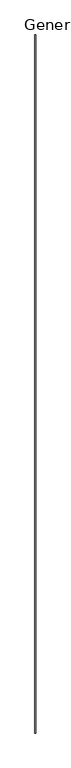
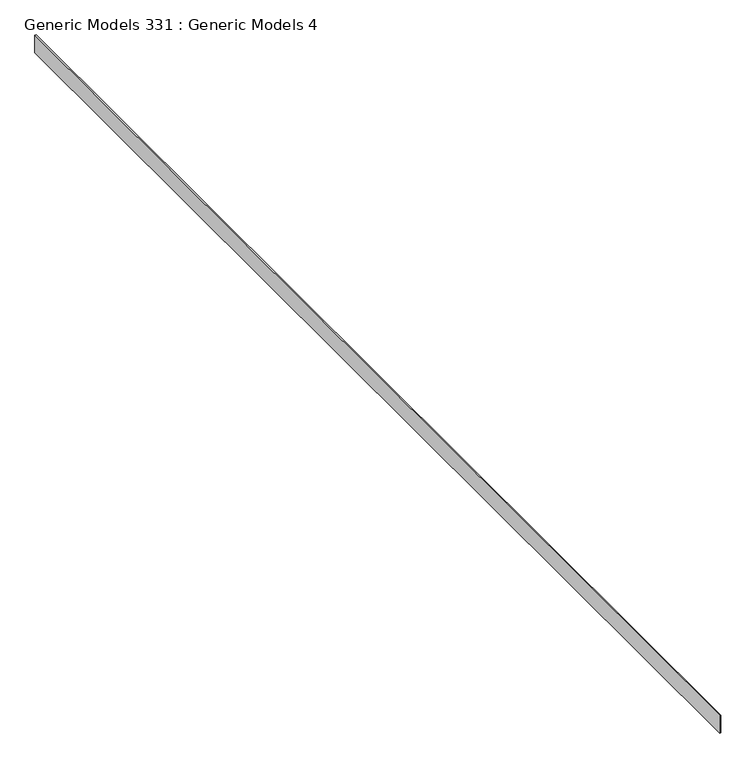
"""IFC4 building model written with IfcOpenShell, lengths in millimetres: proxy geometry, Generic Models 331 : Generic Models 4."""

from ifc_helpers import new_model, si_unit, frame, origin, place, context, project, spatial, polyline, outline, extrude, source, transform, mapped, element, save


def generic_models_331_generic_models_4_b2be233a(model_context):
    return source(origin(), model_context, "Body", "SweptSolid", [
        extrude(outline(polyline([(26420.1627812, 26848.7591064), (26401.1127812, 26848.7591064), (26401.1127812, 45492.3591064), (26420.1627812, 45492.3591064), (26420.1627812, 26848.7591064)])), frame((0.0, 0.0, 130596.677731), z_axis=(0.0, 0.0, 1.0), x_axis=(1.0, 0.0, 0.0)), (0.0, 0.0, 1.0), 293.6073068),
    ])


if __name__ == "__main__":
    model = new_model("IFC4")
    model_context = context("Model", 3, world=origin())
    ifc_project = project(units=[si_unit("LENGTHUNIT", "METRE", prefix="MILLI")], contexts=[model_context])
    site = spatial("IfcSite", under=ifc_project)
    building = spatial("IfcBuilding", under=site)
    placement = place(None, origin())
    generic_models_331_generic_models_4_shape = generic_models_331_generic_models_4_b2be233a(model_context)
    element("IfcBuildingElementProxy", 1, Name="Generic Models 331 : Generic Models 4", ObjectType="Generic Models 331 : Generic Models 4", at=placement, inside=building, context=model_context, shape_type="MappedRepresentation", body=[
        mapped(generic_models_331_generic_models_4_shape, transform((0.0, 0.0, 0.0), x_axis=(1.0, 0.0, 0.0), y_axis=(0.0, 1.0, 0.0), z_axis=(0.0, 0.0, 1.0))),
    ])
    save(model, "model.ifc")

# Revit data of these elements
# Element 1 (IfcBuildingElementProxy, "Generic Models 331 : Generic Models 4")
#   Materials on its faces: "_CDX PLYWOOD - SEE STRUCT DWGs"
# Materials
#   "_CDX PLYWOOD - SEE STRUCT DWGs": class "Generic", colour RGB 98 75 74, transparency 0, Cost = 0
